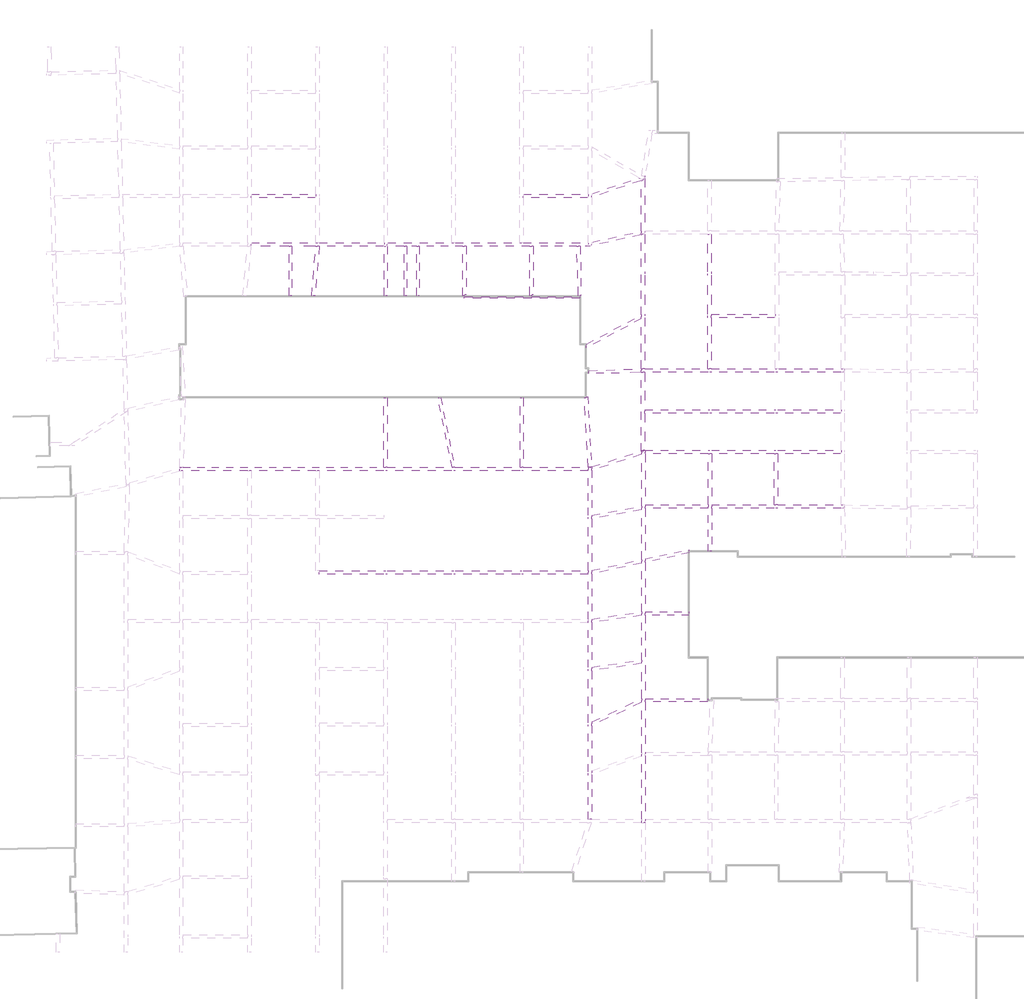
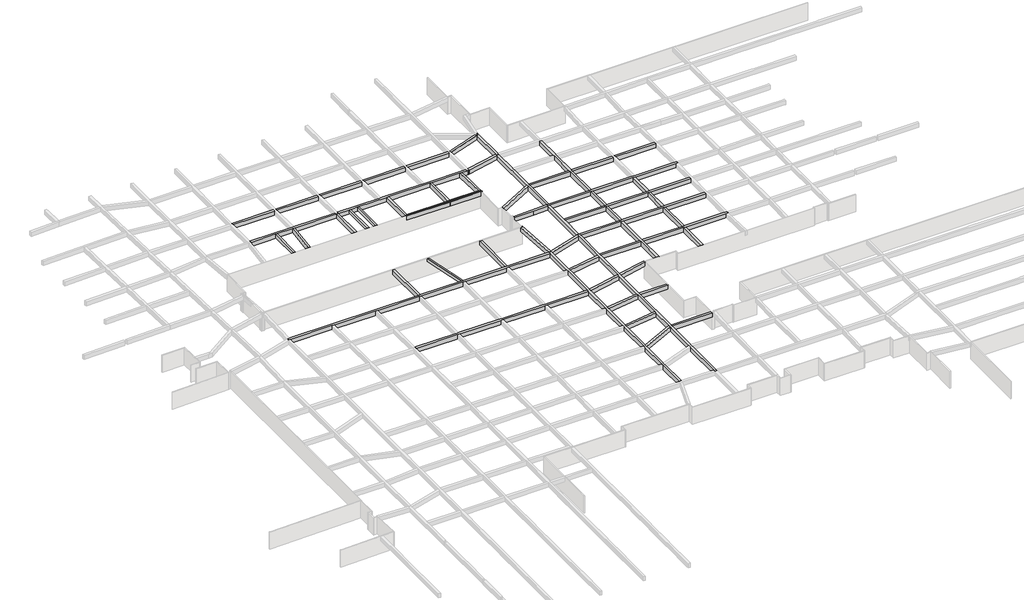
# One storey, part 12 of 20: 47 beams.
# Revit data of these elements (continued)
# Type "混凝土 - 矩形梁 : KL_beam"
#   Length [instance default] = 1524 mm
#   b = 400 mm
#   h = 800 mm
#   Structural Material [instance default] = 混凝土 - 现场浇注混凝土
#   Assembly Code = ""
# Type "混凝土 - 矩形梁 : L_beam"
#   Length [instance default] = 1524 mm
#   b = 300 mm
#   h = 600 mm
#   Structural Material [instance default] = none
#   Assembly Code = ""
# Elements 1, 2, 3, 4, 5, 6, 7, 8, 9, 10, 11, 12, 13, 14, 15, 16, 17, 18, 19, 20, 21, 22, 23, 24, 25, 26, 27, 28, 29, 30, 31, 32, 33, 34, 35, 36, 37, 38, 39, 40, 41, 42, 43 (IfcBeam, "混凝土 - 矩形梁 : KL_beam")
#   Comments = ""
#   Structural Material = none
#   Phase Created = 新构造
# Elements 44, 45, 46, 47 (IfcBeam, "混凝土 - 矩形梁 : L_beam")
#   Comments = ""
#   Structural Material = none
#   Phase Created = 新构造
# Materials
#   "混凝土 - 现场浇注混凝土": class "混凝土", colour RGB 192 192 192, transparency 0
